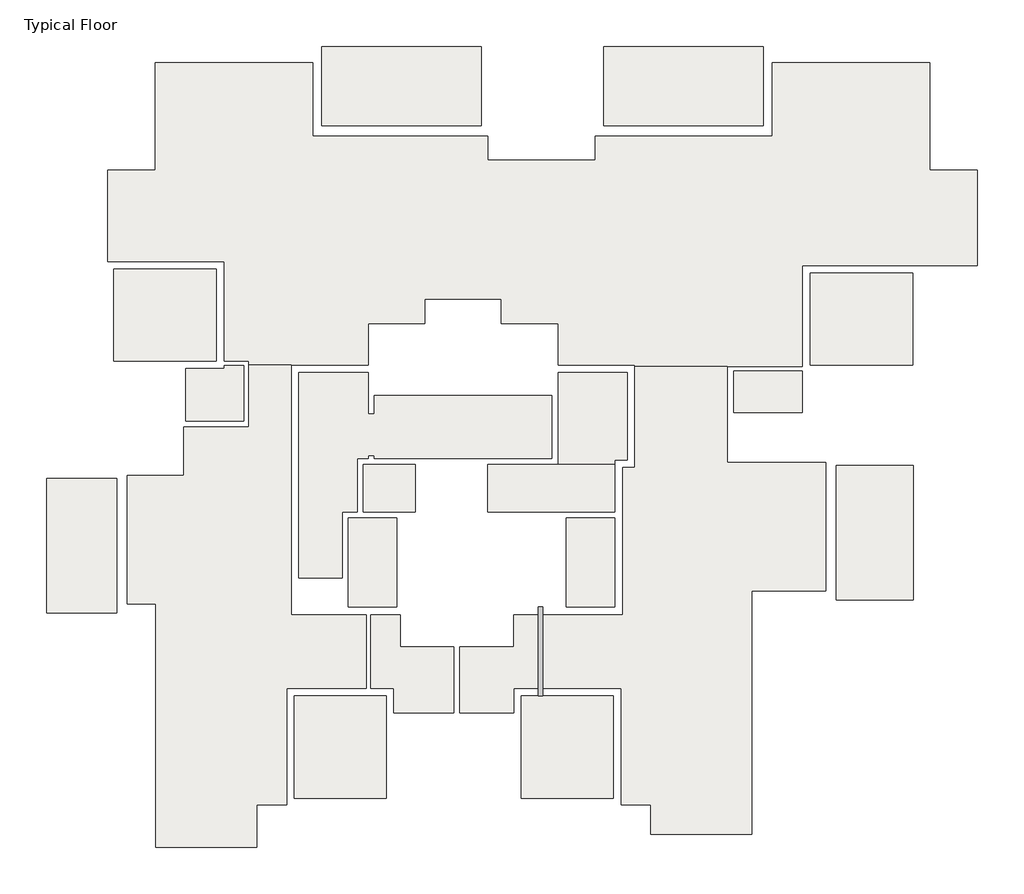
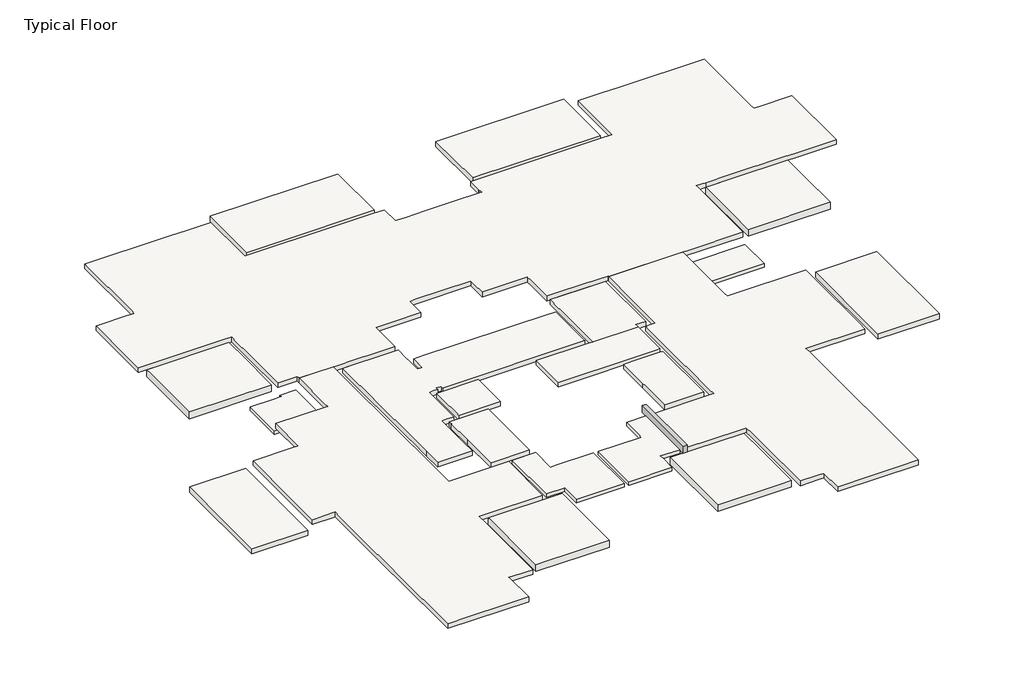
# One storey: 21 slabs, 1 beam.
"""IFC4 building model written with IfcOpenShell, lengths in millimetres."""

from ifc_helpers import new_model, si_unit, frame, origin, place, context, project, spatial, polyline, outline, extrude, faceted_brep, element, save

model = new_model("IFC4")

# Units and contexts
model_context = context("Model", 3, world=origin())
ifc_project = project(units=[si_unit("LENGTHUNIT", "METRE", prefix="MILLI")], contexts=[model_context])

# Site, building, storey
site = spatial("IfcSite", under=ifc_project)
building = spatial("IfcBuilding", under=site)
storey = spatial("IfcBuildingStorey", under=building, Name="Typical Floor", Elevation=3150.0)

# Beam
placement = place(None, origin())
element("IfcBeam", 1, ObjectType="Concrete Rectengular Beam : 15/60", at=placement, inside=storey, context=model_context, shape_type="Brep", body=[
    faceted_brep([(-12635.911942, -10778.5353827, 3450.0), (-12485.911942, -10778.5353827, 3450.0), (-12485.911942, -7874.1201217, 3450.0), (-12635.911942, -7874.1201217, 3450.0), (-12485.911942, -10778.5353827, 3150.0), (-12485.911942, -10528.5353827, 3150.0), (-12485.911942, -10528.5353827, 2950.0), (-12485.911942, -10528.5353827, 2850.0), (-12485.911942, -8124.1201217, 2850.0), (-12485.911942, -8124.1201217, 2950.0), (-12485.911942, -8124.1201217, 3150.0), (-12485.911942, -7874.1201217, 3150.0), (-12635.911942, -10528.5353827, 2850.0), (-12635.911942, -8124.1201217, 2850.0), (-12635.911942, -7874.1201217, 3150.0), (-12635.911942, -8124.1201217, 3150.0), (-12635.911942, -8124.1201217, 3000.0), (-12635.911942, -10528.5353827, 3000.0), (-12635.911942, -10528.5353827, 3150.0), (-12635.911942, -10778.5353827, 3150.0)], [[[0, 1, 2, 3]], [[2, 1, 4, 5, 6, 7, 8, 9, 10, 11]], [[7, 12, 13, 8]], [[0, 3, 14, 15, 16, 13, 12, 17, 18, 19]], [[1, 0, 19, 4]], [[3, 2, 11, 14]], [[5, 18, 17, 12, 7, 6]], [[18, 5, 4, 19]], [[15, 10, 9, 8, 13, 16]], [[10, 15, 14, 11]]]),
])

# Slabs
element("IfcSlab", 2, ObjectType="15", at=placement, inside=storey, context=model_context, shape_type="SweptSolid", body=[
    extrude(outline(polyline([(-3995.4992849, -160.4554551), (-3995.4992849, -1513.3876412), (-6249.3881109, -1513.3876412), (-6249.3881109, -160.4554551), (-3995.4992849, -160.4554551)])), frame((0.0, 0.0, 2550.0), z_axis=(0.0, 0.0, 1.0), x_axis=(1.0, 0.0, 0.0)), (0.0, 0.0, 1.0), 150.0),
])
element("IfcSlab", 3, ObjectType="15", at=placement, inside=storey, context=model_context, shape_type="Brep", body=[
    faceted_brep([(-22902.2127458, -79.7184462, 2550.0), (-22902.2127458, 20.2815538, 2550.0), (-22250.9487358, 20.2815538, 2550.0), (-22250.9487358, -1784.190313, 2550.0), (-24160.0622873, -1784.190313, 2550.0), (-24160.0622873, -79.7184462, 2550.0), (-23152.2127458, -79.7184462, 2550.0), (-22902.2127458, 20.2815538, 2700.0), (-22902.2127458, -79.7184462, 2700.0), (-23152.2127458, -79.7184462, 2700.0), (-24160.0622873, -79.7184462, 2700.0), (-24160.0622873, -1784.190313, 2700.0), (-22250.9487358, -1784.190313, 2700.0), (-22250.9487358, 20.2815538, 2700.0)], [[[0, 1, 2, 3, 4, 5, 6]], [[7, 8, 9, 10, 11, 12, 13]], [[8, 0, 6, 5, 10, 9]], [[1, 0, 8, 7]], [[2, 1, 7, 13]], [[3, 2, 13, 12]], [[4, 3, 12, 11]], [[5, 4, 11, 10]]]),
])
element("IfcSlab", 4, ObjectType="15", at=placement, inside=storey, context=model_context, shape_type="Brep", body=[
    faceted_brep([(-17147.6559701, -8124.1201217, 3000.0), (-17147.6559701, -9176.0843468, 3000.0), (-16947.6559701, -9176.0843468, 3000.0), (-15389.5217009, -9176.0843468, 3000.0), (-15389.5217009, -11338.1261219, 3000.0), (-17348.1541021, -11338.1261219, 3000.0), (-17348.1541021, -10778.5353827, 3000.0), (-17348.1541021, -10528.5353827, 3000.0), (-18103.1541021, -10528.5353827, 3000.0), (-18103.1541021, -8124.1201217, 3000.0), (-17147.6559701, -9176.0843468, 3150.0), (-17147.6559701, -8124.1201217, 3150.0), (-18103.1541021, -8124.1201217, 3150.0), (-18103.1541021, -10528.5353827, 3150.0), (-17348.1541021, -10528.5353827, 3150.0), (-17348.1541021, -10778.5353827, 3150.0), (-17348.1541021, -11338.1261219, 3150.0), (-15389.5217009, -11338.1261219, 3150.0), (-15389.5217009, -9176.0843468, 3150.0), (-16947.6559701, -9176.0843468, 3150.0)], [[[0, 1, 2, 3, 4, 5, 6, 7, 8, 9]], [[10, 11, 12, 13, 14, 15, 16, 17, 18, 19]], [[1, 0, 11, 10]], [[1, 10, 19, 18, 3, 2]], [[4, 3, 18, 17]], [[5, 4, 17, 16]], [[5, 16, 15, 14, 7, 6]], [[8, 7, 14, 13]], [[9, 8, 13, 12]], [[0, 9, 12, 11]]]),
])
element("IfcSlab", 5, ObjectType="15", at=placement, inside=storey, context=model_context, shape_type="Brep", body=[
    faceted_brep([(-12635.911942, -8124.1201217, 3000.0), (-12635.911942, -10528.5353827, 3000.0), (-13430.911942, -10528.5353827, 3000.0), (-13430.911942, -10778.5353827, 3000.0), (-13430.911942, -11338.1261219, 3000.0), (-15189.5217009, -11338.1261219, 3000.0), (-15189.5217009, -9176.0843468, 3000.0), (-13431.410074, -9176.0843468, 3000.0), (-13431.410074, -8976.0843468, 3000.0), (-13431.410074, -8124.1201217, 3000.0), (-12635.911942, -10528.5353827, 3150.0), (-12635.911942, -8124.1201217, 3150.0), (-13431.410074, -8124.1201217, 3150.0), (-13431.410074, -8976.0843468, 3150.0), (-13431.410074, -9176.0843468, 3150.0), (-15189.5217009, -9176.0843468, 3150.0), (-15189.5217009, -11338.1261219, 3150.0), (-13430.911942, -11338.1261219, 3150.0), (-13430.911942, -10778.5353827, 3150.0), (-13430.911942, -10528.5353827, 3150.0)], [[[0, 1, 2, 3, 4, 5, 6, 7, 8, 9]], [[10, 11, 12, 13, 14, 15, 16, 17, 18, 19]], [[1, 0, 11, 10]], [[2, 1, 10, 19]], [[2, 19, 18, 17, 4, 3]], [[5, 4, 17, 16]], [[6, 5, 16, 15]], [[7, 6, 15, 14]], [[7, 14, 13, 12, 9, 8]], [[0, 9, 12, 11]]]),
])
element("IfcSlab", 6, ObjectType="20", at=placement, inside=storey, context=model_context, shape_type="Brep", body=[
    faceted_brep([(-14287.2982207, 7522.5061661, 2950.0), (-14287.2982207, 6745.5504319, 2950.0), (-10767.128403, 6745.5504319, 2950.0), (-10767.128403, 6945.5504319, 2950.0), (-10767.6095532, 6945.5504319, 2950.0), (-10767.6095532, 7522.0250158, 2950.0), (-10278.642045, 7522.0250158, 2950.0), (-7273.2531624, 7522.0250158, 2950.0), (-6464.4905676, 7522.0250158, 2950.0), (-5362.5320031, 7522.0250158, 2950.0), (-4977.1589702, 7522.0250158, 2950.0), (-4977.1589702, 7872.0250158, 2950.0), (-4977.1589702, 9926.4176344, 2950.0), (161.8198592, 9926.4176344, 2950.0), (161.8198592, 6620.0664514, 2950.0), (161.3217272, 6620.0664514, 2950.0), (161.3217272, 6420.0664514, 2950.0), (1724.6637401, 6420.0664514, 2950.0), (1724.6637401, 3294.4013319, 2950.0), (11.338709, 3294.4013319, 2950.0), (-388.661291, 3294.4013319, 2950.0), (-2382.6064399, 3294.4013319, 2950.0), (-2675.3362599, 3294.4013319, 2950.0), (-3574.7135949, 3294.4013319, 2950.0), (-3574.7135949, 3294.8994639, 2950.0), (-3995.4992849, 3294.8994639, 2950.0), (-3995.4992849, 3044.8994639, 2950.0), (-3995.4992849, -10.4554551, 2950.0), (-6449.3881109, -10.4554551, 2950.0), (-9474.5664195, -10.4554551, 2950.0), (-9474.5664195, 39.0464129, 2950.0), (-10476.5363052, 39.0464129, 2950.0), (-11477.9854165, 39.0464129, 2950.0), (-11984.1625168, 39.0464129, 2950.0), (-11984.1625168, 1141.4974488, 2950.0), (-11984.1625168, 1391.4974488, 2950.0), (-13837.0933073, 1391.4974488, 2950.0), (-13837.0933073, 1942.9408995, 2950.0), (-13837.0933073, 2192.9408995, 2950.0), (-16091.0047757, 2192.9408995, 2950.0), (-16341.0047757, 2192.9408995, 2950.0), (-16341.0047757, 1391.4691458, 2950.0), (-17944.4124515, 1391.4691458, 2950.0), (-18194.4124515, 1391.4691458, 2950.0), (-18194.4124515, 39.5388843, 2950.0), (-18915.6849523, 39.5388843, 2950.0), (-19917.1340636, 39.5388843, 2950.0), (-20453.5033605, 39.5388843, 2950.0), (-20703.5033605, 39.5388843, 2950.0), (-22100.9487358, 39.5388843, 2950.0), (-22100.9487358, 170.2815538, 2950.0), (-22902.2127458, 170.2815538, 2950.0), (-22902.2127458, 2208.0433561, 2950.0), (-22902.2127458, 3085.0930561, 2950.0), (-22902.2127458, 3425.0930561, 2950.0), (-23152.2127458, 3425.0930561, 2950.0), (-26709.0507397, 3425.0930561, 2950.0), (-26709.0507397, 6420.0664514, 2950.0), (-26578.3590155, 6420.0664514, 2950.0), (-25426.4061116, 6420.0664514, 2950.0), (-25146.2068588, 6420.0664514, 2950.0), (-25146.2068588, 6620.0664514, 2950.0), (-25146.2068588, 9925.9195024, 2950.0), (-24284.8686951, 9925.9195024, 2950.0), (-22681.9251878, 9925.9195024, 2950.0), (-21629.9609627, 9925.9195024, 2950.0), (-20978.9930017, 9925.9195024, 2950.0), (-20006.7412186, 9925.9195024, 2950.0), (-20006.7412186, 7872.5061661, 2950.0), (-20006.7412186, 7522.5061661, 2950.0), (-19621.8549965, 7522.5061661, 2950.0), (-18519.896432, 7522.5061661, 2950.0), (-17711.1338372, 7522.5061661, 2950.0), (-14706.2657289, 7522.5061661, 2950.0), (-14287.2982207, 6745.5504319, 3150.0), (-14287.2982207, 7522.5061661, 3150.0), (-14706.2657289, 7522.5061661, 3150.0), (-17711.1338372, 7522.5061661, 3150.0), (-18519.896432, 7522.5061661, 3150.0), (-19621.8549965, 7522.5061661, 3150.0), (-20006.7412186, 7522.5061661, 3150.0), (-20006.7412186, 7872.5061661, 3150.0), (-20006.7412186, 9925.9195024, 3150.0), (-20978.9930017, 9925.9195024, 3150.0), (-21629.9609627, 9925.9195024, 3150.0), (-22681.9251878, 9925.9195024, 3150.0), (-24284.8686951, 9925.9195024, 3150.0), (-25146.2068588, 9925.9195024, 3150.0), (-25146.2068588, 6620.0664514, 3150.0), (-25146.2068588, 6420.0664514, 3150.0), (-25426.4061116, 6420.0664514, 3150.0), (-26578.3590155, 6420.0664514, 3150.0), (-26709.0507397, 6420.0664514, 3150.0), (-26709.0507397, 3425.0930561, 3150.0), (-23152.2127458, 3425.0930561, 3150.0), (-22902.2127458, 3425.0930561, 3150.0), (-22902.2127458, 3085.0930561, 3150.0), (-22902.2127458, 2208.0433561, 3150.0), (-22902.2127458, 170.2815538, 3150.0), (-22100.9487358, 170.2815538, 3150.0), (-22100.9487358, 39.5388843, 3150.0), (-20703.5033605, 39.5388843, 3150.0), (-20453.5033605, 39.5388843, 3150.0), (-19917.1340636, 39.5388843, 3150.0), (-18915.6849523, 39.5388843, 3150.0), (-18194.4124515, 39.5388843, 3150.0), (-18194.4124515, 1391.4691458, 3150.0), (-17944.4124515, 1391.4691458, 3150.0), (-16341.0047757, 1391.4691458, 3150.0), (-16341.0047757, 2192.9408995, 3150.0), (-16091.0047757, 2192.9408995, 3150.0), (-13837.0933073, 2192.9408995, 3150.0), (-13837.0933073, 1942.9408995, 3150.0), (-13837.0933073, 1391.4974488, 3150.0), (-11984.1625168, 1391.4974488, 3150.0), (-11984.1625168, 1141.4974488, 3150.0), (-11984.1625168, 39.0464129, 3150.0), (-11477.9854165, 39.0464129, 3150.0), (-10476.5363052, 39.0464129, 3150.0), (-9474.5664195, 39.0464129, 3150.0), (-9474.5664195, -10.4554551, 3150.0), (-6449.3881109, -10.4554551, 3150.0), (-6249.3881109, -10.4554551, 3150.0), (-3995.4992849, -10.4554551, 3150.0), (-3995.4992849, 3044.8994639, 3150.0), (-3995.4992849, 3294.8994639, 3150.0), (-3574.7135949, 3294.8994639, 3150.0), (-3574.7135949, 3294.4013319, 3150.0), (-2675.3362599, 3294.4013319, 3150.0), (-388.661291, 3294.4013319, 3150.0), (11.338709, 3294.4013319, 3150.0), (1724.6637401, 3294.4013319, 3150.0), (1724.6637401, 6420.0664514, 3150.0), (1593.9720159, 6420.0664514, 3150.0), (442.019112, 6420.0664514, 3150.0), (161.3217272, 6420.0664514, 3150.0), (161.3217272, 6620.0664514, 3150.0), (161.8198592, 6620.0664514, 3150.0), (161.8198592, 9926.4176344, 3150.0), (-700.0390789, 9926.4176344, 3150.0), (-2302.4618118, 9926.4176344, 3150.0), (-3354.4260369, 9926.4176344, 3150.0), (-4005.3939979, 9926.4176344, 3150.0), (-4977.1589702, 9926.4176344, 3150.0), (-4977.1589702, 7872.0250158, 3150.0), (-4977.1589702, 7522.0250158, 3150.0), (-5362.5320031, 7522.0250158, 3150.0), (-6464.4905676, 7522.0250158, 3150.0), (-7273.2531624, 7522.0250158, 3150.0), (-10278.642045, 7522.0250158, 3150.0), (-10767.6095532, 7522.0250158, 3150.0), (-10767.6095532, 6945.5504319, 3150.0), (-10767.128403, 6945.5504319, 3150.0), (-10767.128403, 6745.5504319, 3150.0), (-11941.4746047, 6745.5504319, 3150.0), (-13043.4331692, 6745.5504319, 3150.0), (-13867.2982207, 6745.5504319, 3150.0), (-3574.7135949, 3294.4013319, 3100.0)], [[[0, 1, 2, 3, 4, 5, 6, 7, 8, 9, 10, 11, 12, 13, 14, 15, 16, 17, 18, 19, 20, 21, 22, 23, 24, 25, 26, 27, 28, 29, 30, 31, 32, 33, 34, 35, 36, 37, 38, 39, 40, 41, 42, 43, 44, 45, 46, 47, 48, 49, 50, 51, 52, 53, 54, 55, 56, 57, 58, 59, 60, 61, 62, 63, 64, 65, 66, 67, 68, 69, 70, 71, 72, 73]], [[74, 75, 76, 77, 78, 79, 80, 81, 82, 83, 84, 85, 86, 87, 88, 89, 90, 91, 92, 93, 94, 95, 96, 97, 98, 99, 100, 101, 102, 103, 104, 105, 106, 107, 108, 109, 110, 111, 112, 113, 114, 115, 116, 117, 118, 119, 120, 121, 122, 123, 124, 125, 126, 127, 128, 129, 130, 131, 132, 133, 134, 135, 136, 137, 138, 139, 140, 141, 142, 143, 144, 145, 146, 147, 148, 149, 150, 151, 152, 153, 154, 155, 156]], [[89, 60, 59, 58, 57, 92, 91, 90]], [[60, 89, 88, 87, 62, 61]], [[62, 87, 86, 85, 84, 83, 82, 67, 66, 65, 64, 63]], [[67, 82, 81, 80, 69, 68]], [[69, 80, 79, 78, 77, 76, 75, 0, 73, 72, 71, 70]], [[1, 0, 75, 74]], [[1, 74, 156, 155, 154, 153, 2]], [[150, 5, 4, 151]], [[6, 5, 150, 149]], [[6, 149, 148, 147, 146, 145, 10, 9, 8, 7]], [[10, 145, 144, 143, 12, 11]], [[13, 12, 143, 142, 141, 140, 139, 138]], [[13, 138, 137, 14]], [[132, 17, 16, 135, 134, 133]], [[18, 17, 132, 131]], [[18, 131, 130, 129, 128, 127, 157, 23, 22, 21, 20, 19]], [[123, 27, 26, 25, 125, 124]], [[28, 27, 123, 122, 121]], [[29, 28, 121, 120]], [[30, 29, 120, 119]], [[30, 119, 118, 117, 116, 33, 32, 31]], [[33, 116, 115, 114, 35, 34]], [[36, 35, 114, 113]], [[36, 113, 112, 111, 38, 37]], [[38, 111, 110, 109, 40, 39]], [[41, 40, 109, 108]], [[41, 108, 107, 106, 43, 42]], [[44, 43, 106, 105]], [[44, 105, 104, 103, 102, 101, 48, 47, 46, 45]], [[49, 48, 101, 100]], [[50, 49, 100, 99]], [[51, 50, 99, 98]], [[51, 98, 97, 96, 95, 54, 53, 52]], [[54, 95, 94, 93, 56, 55]], [[57, 56, 93, 92]], [[24, 126, 125, 25]], [[126, 24, 23, 157, 127]], [[3, 152, 151, 4]], [[2, 153, 152, 3]], [[136, 15, 14, 137]], [[135, 16, 15, 136]]]),
])
element("IfcSlab", 7, ObjectType="20", at=placement, inside=storey, context=model_context, shape_type="Brep", body=[
    faceted_brep([(-3237.9389996, -3145.5397979, 2950.0), (-3237.9389996, -7343.0129016, 2950.0), (-5648.4371316, -7343.0129016, 2950.0), (-5648.4371316, -7643.0129016, 2950.0), (-5648.4371316, -8389.7150498, 2950.0), (-5648.4371316, -9591.6622931, 2950.0), (-5648.4371316, -11149.2984303, 2950.0), (-5648.4371316, -11806.6175745, 2950.0), (-5648.4371316, -15307.4032645, 2950.0), (-8953.7920507, -15307.4032645, 2950.0), (-8953.7920507, -14334.8752446, 2950.0), (-9153.7920507, -14334.8752446, 2950.0), (-9925.0588909, -14334.8752446, 2950.0), (-9925.0588909, -11794.8752446, 2950.0), (-9925.0588909, -10898.8059589, 2950.0), (-9925.0588909, -10528.5353827, 2950.0), (-10175.0588909, -10528.5353827, 2950.0), (-12485.911942, -10528.5353827, 2950.0), (-12485.911942, -8124.1201217, 2950.0), (-9876.055155, -8124.1201217, 2950.0), (-9876.055155, -7874.1201217, 2950.0), (-9876.055155, -4468.2840524, 2950.0), (-9876.055155, -3466.3141668, 2950.0), (-9876.055155, -3316.3311485, 2950.0), (-9724.5664195, -3316.3311485, 2950.0), (-9474.5664195, -3316.3311485, 2950.0), (-9474.5664195, -210.9535871, 2950.0), (-9474.5664195, -10.4554551, 2950.0), (-6449.3881109, -10.4554551, 2950.0), (-6449.3881109, -1513.3876412, 2950.0), (-6449.3881109, -1713.3876412, 2950.0), (-6449.3881109, -2845.5511191, 2950.0), (-6449.3881109, -3145.5397979, 2950.0), (-6249.3881109, -3145.5397979, 2950.0), (-3237.9389996, -7343.0129016, 3150.0), (-3237.9389996, -6903.0129016, 3150.0), (-3237.9389996, -3892.3076005, 3150.0), (-3237.9389996, -3145.5397979, 3150.0), (-6249.3881109, -3145.5397979, 3150.0), (-6449.3881109, -3145.5397979, 3150.0), (-6449.3881109, -2845.5511191, 3150.0), (-6449.3881109, -1713.3876412, 3150.0), (-6449.3881109, -1513.3876412, 3150.0), (-6449.3881109, -10.4554551, 3150.0), (-9474.5664195, -10.4554551, 3150.0), (-9474.5664195, -210.9535871, 3150.0), (-9474.5664195, -3316.3311485, 3150.0), (-9724.5664195, -3316.3311485, 3150.0), (-9876.055155, -3316.3311485, 3150.0), (-9876.055155, -3466.3141668, 3150.0), (-9876.055155, -4468.2840524, 3150.0), (-9876.055155, -7874.1201217, 3150.0), (-9876.055155, -8124.1201217, 3150.0), (-12485.911942, -8124.1201217, 3150.0), (-12485.911942, -10528.5353827, 3150.0), (-10175.0588909, -10528.5353827, 3150.0), (-9925.0588909, -10528.5353827, 3150.0), (-9925.0588909, -10898.8059589, 3150.0), (-9925.0588909, -11794.8752446, 3150.0), (-9925.0588909, -14334.8752446, 3150.0), (-9153.7920507, -14334.8752446, 3150.0), (-8953.7920507, -14334.8752446, 3150.0), (-8953.7920507, -15307.4032645, 3150.0), (-8093.7920507, -15307.4032645, 3150.0), (-6499.9032247, -15307.4032645, 3150.0), (-5648.4371316, -15307.4032645, 3150.0), (-5648.4371316, -11806.6175745, 3150.0), (-5648.4371316, -11149.2984303, 3150.0), (-5648.4371316, -9591.6622931, 3150.0), (-5648.4371316, -8389.7150498, 3150.0), (-5648.4371316, -7643.0129016, 3150.0), (-5648.4371316, -7343.0129016, 3150.0)], [[[0, 1, 2, 3, 4, 5, 6, 7, 8, 9, 10, 11, 12, 13, 14, 15, 16, 17, 18, 19, 20, 21, 22, 23, 24, 25, 26, 27, 28, 29, 30, 31, 32, 33]], [[34, 35, 36, 37, 38, 39, 40, 41, 42, 43, 44, 45, 46, 47, 48, 49, 50, 51, 52, 53, 54, 55, 56, 57, 58, 59, 60, 61, 62, 63, 64, 65, 66, 67, 68, 69, 70, 71]], [[39, 32, 31, 30, 29, 28, 43, 42, 41, 40]], [[32, 39, 38, 37, 0, 33]], [[1, 0, 37, 36, 35, 34]], [[2, 1, 34, 71]], [[2, 71, 70, 69, 68, 67, 66, 65, 8, 7, 6, 5, 4, 3]], [[9, 8, 65, 64, 63, 62]], [[10, 9, 62, 61]], [[10, 61, 60, 59, 12, 11]], [[12, 59, 58, 57, 56, 15, 14, 13]], [[15, 56, 55, 54, 17, 16]], [[18, 17, 54, 53]], [[19, 18, 53, 52]], [[19, 52, 51, 50, 49, 48, 23, 22, 21, 20]], [[23, 48, 47, 46, 25, 24]], [[25, 46, 45, 44, 27, 26]], [[28, 27, 44, 43]]]),
])
element("IfcSlab", 8, ObjectType="20", at=placement, inside=storey, context=model_context, shape_type="Brep", body=[
    faceted_brep([(-18253.1541021, -8124.1201217, 2950.0), (-18253.1541021, -10528.5353827, 2950.0), (-20604.0071531, -10528.5353827, 2950.0), (-20854.0071531, -10528.5353827, 2950.0), (-20854.0071531, -10898.8059589, 2950.0), (-20854.0071531, -11794.8752446, 2950.0), (-20854.0071531, -14334.8752446, 2950.0), (-21625.2739934, -14334.8752446, 2950.0), (-21825.2739934, -14334.8752446, 2950.0), (-21825.2739934, -15727.4032645, 2950.0), (-25131.1270445, -15727.4032645, 2950.0), (-25131.1270445, -12221.0520814, 2950.0), (-25131.1270445, -11570.0841204, 2950.0), (-25131.1270445, -10012.4479831, 2950.0), (-25131.1270445, -8810.5007399, 2950.0), (-25131.1270445, -8064.2310693, 2950.0), (-25131.1270445, -7764.2310693, 2950.0), (-26062.7923903, -7764.2310693, 2950.0), (-26062.7923903, -3566.82362, 2950.0), (-24415.0622873, -3566.82362, 2950.0), (-24215.0622873, -3566.82362, 2950.0), (-24215.0622873, -1984.190313, 2950.0), (-22100.9487358, -1984.190313, 2950.0), (-22100.9487358, -1784.190313, 2950.0), (-22100.9487358, 39.5388843, 2950.0), (-20703.5033605, 39.5388843, 2950.0), (-20703.5033605, -5109.3573005, 2950.0), (-20703.0108891, -5109.3573005, 2950.0), (-20703.0108891, -6110.8064118, 2950.0), (-20703.0108891, -7874.1201217, 2950.0), (-20703.5033605, -7874.1201217, 2950.0), (-20703.5033605, -8124.1201217, 2950.0), (-18253.1541021, -10528.5353827, 3150.0), (-18253.1541021, -8124.1201217, 3150.0), (-20703.5033605, -8124.1201217, 3150.0), (-20703.5033605, -7874.1201217, 3150.0), (-20703.0108891, -7874.1201217, 3150.0), (-20703.0108891, -6110.8064118, 3150.0), (-20703.0108891, -5109.3573005, 3150.0), (-20703.5033605, -5109.3573005, 3150.0), (-20703.5033605, 39.5388843, 3150.0), (-22100.9487358, 39.5388843, 3150.0), (-22100.9487358, -1784.190313, 3150.0), (-22100.9487358, -1984.190313, 3150.0), (-24215.0622873, -1984.190313, 3150.0), (-24215.0622873, -3566.82362, 3150.0), (-24415.0622873, -3566.82362, 3150.0), (-26062.7923903, -3566.82362, 3150.0), (-26062.7923903, -4267.7859204, 3150.0), (-26062.7923903, -7272.6540287, 3150.0), (-26062.7923903, -7764.2310693, 3150.0), (-25131.1270445, -7764.2310693, 3150.0), (-25131.1270445, -8064.2310693, 3150.0), (-25131.1270445, -8810.5007399, 3150.0), (-25131.1270445, -10012.4479831, 3150.0), (-25131.1270445, -11570.0841204, 3150.0), (-25131.1270445, -12221.0520814, 3150.0), (-25131.1270445, -15727.4032645, 3150.0), (-24279.6609514, -15727.4032645, 3150.0), (-22676.7174441, -15727.4032645, 3150.0), (-21825.2739934, -15727.4032645, 3150.0), (-21825.2739934, -14334.8752446, 3150.0), (-21625.2739934, -14334.8752446, 3150.0), (-20854.0071531, -14334.8752446, 3150.0), (-20854.0071531, -11794.8752446, 3150.0), (-20854.0071531, -10898.8059589, 3150.0), (-20854.0071531, -10528.5353827, 3150.0), (-20604.0071531, -10528.5353827, 3150.0), (-20703.0108891, -5109.3573005, 3050.0)], [[[0, 1, 2, 3, 4, 5, 6, 7, 8, 9, 10, 11, 12, 13, 14, 15, 16, 17, 18, 19, 20, 21, 22, 23, 24, 25, 26, 27, 28, 29, 30, 31]], [[32, 33, 34, 35, 36, 37, 38, 39, 40, 41, 42, 43, 44, 45, 46, 47, 48, 49, 50, 51, 52, 53, 54, 55, 56, 57, 58, 59, 60, 61, 62, 63, 64, 65, 66, 67]], [[24, 41, 40, 25]], [[36, 29, 28, 27, 68, 38, 37]], [[33, 0, 31, 34]], [[1, 0, 33, 32]], [[1, 32, 67, 66, 3, 2]], [[3, 66, 65, 64, 63, 6, 5, 4]], [[6, 63, 62, 61, 8, 7]], [[9, 8, 61, 60]], [[10, 9, 60, 59, 58, 57]], [[10, 57, 56, 55, 54, 53, 52, 51, 16, 15, 14, 13, 12, 11]], [[17, 16, 51, 50]], [[18, 17, 50, 49, 48, 47]], [[18, 47, 46, 45, 20, 19]], [[21, 20, 45, 44]], [[22, 21, 44, 43]], [[22, 43, 42, 41, 24, 23]], [[35, 30, 29, 36]], [[34, 31, 30, 35]], [[39, 26, 25, 40]], [[26, 39, 38, 68, 27]]]),
])
element("IfcSlab", 9, ObjectType="20", at=placement, inside=storey, context=model_context, shape_type="Brep", body=[
    faceted_brep([(-20453.5033605, -210.4611157, 2950.0), (-18194.4124515, -210.4611157, 2950.0), (-18194.4124515, -762.4310014, 2950.0), (-18194.4124515, -962.4310014, 2950.0), (-18194.4124515, -1563.404623, 2950.0), (-17994.4124515, -1563.404623, 2950.0), (-17994.4124515, -962.4325886, 2950.0), (-17984.178103, -962.4325886, 2950.0), (-17593.4388298, -962.4325886, 2950.0), (-16290.9821333, -962.4325886, 2950.0), (-15740.0028511, -962.4325886, 2950.0), (-14438.066929, -962.4325886, 2950.0), (-13887.0876467, -962.4325886, 2950.0), (-12584.1498, -962.4325886, 2950.0), (-12184.178103, -962.4325886, 2950.0), (-12184.178103, -3015.8216954, 2950.0), (-17993.9143195, -3015.8216954, 2950.0), (-17993.9143195, -2915.3348845, 2950.0), (-18193.9143195, -2915.3348845, 2950.0), (-18193.9143195, -3015.8216954, 2950.0), (-18350.1013454, -3015.8216954, 2950.0), (-18550.1013454, -3015.8216954, 2950.0), (-18550.1013454, -3666.8122988, 2950.0), (-18550.1013454, -4618.2670707, 2950.0), (-18550.1013454, -4768.7708633, 2950.0), (-18843.2746727, -4768.7708633, 2950.0), (-19043.2746727, -4768.7708633, 2950.0), (-19043.2746727, -5119.2520135, 2950.0), (-19043.2746727, -6221.210578, 2950.0), (-19043.2746727, -6922.1728784, 2950.0), (-20453.0108891, -6922.1728784, 2950.0), (-20453.0108891, -6110.8064118, 2950.0), (-20453.5033605, -6110.8064118, 2950.0), (-20453.5033605, -5109.3573005, 2950.0), (-20453.5033605, -4948.7708633, 2950.0), (-18194.4124515, -210.4611157, 3150.0), (-18915.6849523, -210.4611157, 3150.0), (-19917.1340636, -210.4611157, 3150.0), (-20453.5033605, -210.4611157, 3150.0), (-20453.5033605, -5109.3573005, 3150.0), (-20453.5033605, -6110.8064118, 3150.0), (-20453.0108891, -6110.8064118, 3150.0), (-20453.0108891, -6922.1728784, 3150.0), (-19043.2746727, -6922.1728784, 3150.0), (-19043.2746727, -6221.210578, 3150.0), (-19043.2746727, -5119.2520135, 3150.0), (-19043.2746727, -4768.7708633, 3150.0), (-18843.2746727, -4768.7708633, 3150.0), (-18550.1013454, -4768.7708633, 3150.0), (-18550.1013454, -4618.2670707, 3150.0), (-18550.1013454, -3666.8122988, 3150.0), (-18550.1013454, -3015.8216954, 3150.0), (-18350.1013454, -3015.8216954, 3150.0), (-18193.9143195, -3015.8216954, 3150.0), (-18193.9143195, -2915.3348845, 3150.0), (-17993.9143195, -2915.3348845, 3150.0), (-17993.9143195, -3015.8216954, 3150.0), (-12184.178103, -3015.8216954, 3150.0), (-12184.178103, -2915.3348845, 3150.0), (-12184.178103, -1563.404623, 3150.0), (-12184.178103, -962.4325886, 3150.0), (-12584.1498, -962.4325886, 3150.0), (-13887.0876467, -962.4325886, 3150.0), (-14438.066929, -962.4325886, 3150.0), (-15740.0028511, -962.4325886, 3150.0), (-16290.9821333, -962.4325886, 3150.0), (-17593.4388298, -962.4325886, 3150.0), (-17984.178103, -962.4325886, 3150.0), (-17994.4124515, -962.4325886, 3150.0), (-17994.4124515, -1563.404623, 3150.0), (-18194.4124515, -1563.404623, 3150.0), (-18194.4124515, -962.4310014, 3150.0), (-18194.4124515, -762.4310014, 3150.0), (-20453.5033605, -6110.8064118, 3050.0)], [[[0, 1, 2, 3, 4, 5, 6, 7, 8, 9, 10, 11, 12, 13, 14, 15, 16, 17, 18, 19, 20, 21, 22, 23, 24, 25, 26, 27, 28, 29, 30, 31, 32, 33, 34]], [[35, 36, 37, 38, 39, 40, 41, 42, 43, 44, 45, 46, 47, 48, 49, 50, 51, 52, 53, 54, 55, 56, 57, 58, 59, 60, 61, 62, 63, 64, 65, 66, 67, 68, 69, 70, 71, 72]], [[29, 43, 42, 30]], [[38, 0, 34, 33, 32, 73, 40, 39]], [[1, 0, 38, 37, 36, 35]], [[1, 35, 72, 71, 70, 4, 3, 2]], [[5, 4, 70, 69]], [[6, 5, 69, 68]], [[7, 6, 68, 67]], [[7, 67, 66, 65, 64, 63, 62, 61, 60, 14, 13, 12, 11, 10, 9, 8]], [[15, 14, 60, 59, 58, 57]], [[16, 15, 57, 56]], [[17, 16, 56, 55]], [[18, 17, 55, 54]], [[19, 18, 54, 53]], [[19, 53, 52, 51, 21, 20]], [[21, 51, 50, 49, 48, 24, 23, 22]], [[24, 48, 47, 46, 26, 25]], [[26, 46, 45, 44, 43, 29, 28, 27]], [[41, 31, 30, 42]], [[31, 41, 40, 73, 32]]]),
])
element("IfcSlab", 10, ObjectType="20", at=placement, inside=storey, context=model_context, shape_type="Brep", body=[
    faceted_brep([(-16646.6710273, -3215.8216954, 2950.0), (-16646.6710273, -4768.7708633, 2950.0), (-18350.1013454, -4768.7708633, 2950.0), (-18350.1013454, -3215.8216954, 2950.0), (-16646.6710273, -4768.7708633, 3150.0), (-16646.6710273, -3215.8216954, 3150.0), (-18350.1013454, -3215.8216954, 3150.0), (-18350.1013454, -3666.8122988, 3150.0), (-18350.1013454, -4618.2670707, 3150.0), (-18350.1013454, -4768.7708633, 3150.0)], [[[0, 1, 2, 3]], [[4, 5, 6, 7, 8, 9]], [[1, 0, 5, 4]], [[2, 1, 4, 9]], [[3, 2, 9, 8, 7, 6]], [[0, 3, 6, 5]]]),
])
element("IfcSlab", 11, ObjectType="20", at=placement, inside=storey, context=model_context, shape_type="Brep", body=[
    faceted_brep([(-11723.2701442, -4968.7708633, 2950.0), (-10126.055155, -4968.7708633, 2950.0), (-10126.055155, -7874.1201217, 2950.0), (-11723.2701442, -7874.1201217, 2950.0), (-11723.2701442, -6321.6973888, 2950.0), (-10126.055155, -4968.7708633, 3150.0), (-10226.0438338, -4968.7708633, 3150.0), (-11328.0023982, -4968.7708633, 3150.0), (-11723.2701442, -4968.7708633, 3150.0), (-11723.2701442, -6321.6973888, 3150.0), (-11723.2701442, -6521.6973888, 3150.0), (-11723.2701442, -7874.1201217, 3150.0), (-10126.055155, -7874.1201217, 3150.0)], [[[0, 1, 2, 3, 4]], [[5, 6, 7, 8, 9, 10, 11, 12]], [[1, 0, 8, 7, 6, 5]], [[2, 1, 5, 12]], [[3, 2, 12, 11]], [[4, 3, 11, 10, 9]], [[0, 4, 9, 8]]]),
])
element("IfcSlab", 12, ObjectType="20", at=placement, inside=storey, context=model_context, shape_type="Brep", body=[
    faceted_brep([(-17252.8523926, -4968.7708633, 2950.0), (-17252.8523926, -7874.1201217, 2950.0), (-18843.2746727, -7874.1201217, 2950.0), (-18843.2746727, -6221.210578, 2950.0), (-18848.2746727, -6221.210578, 2950.0), (-18848.2746727, -5119.2520135, 2950.0), (-18843.2746727, -5119.2520135, 2950.0), (-18843.2746727, -4968.7708633, 2950.0), (-17252.8523926, -7874.1201217, 3150.0), (-17252.8523926, -4968.7708633, 3150.0), (-18843.2746727, -4968.7708633, 3150.0), (-18843.2746727, -5119.2520135, 3150.0), (-18848.2746727, -5119.2520135, 3150.0), (-18848.2746727, -6221.210578, 3150.0), (-18843.2746727, -6221.210578, 3150.0), (-18843.2746727, -7874.1201217, 3150.0), (-18848.2746727, -5119.2520135, 3050.0), (-18848.2746727, -6221.210578, 3050.0)], [[[0, 1, 2, 3, 4, 5, 6, 7]], [[8, 9, 10, 11, 12, 13, 14, 15]], [[1, 0, 9, 8]], [[1, 8, 15, 2]], [[12, 16, 5, 4, 17, 13]], [[9, 0, 7, 10]], [[6, 11, 10, 7]], [[11, 6, 5, 16, 12]], [[14, 3, 2, 15]], [[3, 14, 13, 17, 4]]]),
])
element("IfcSlab", 13, ObjectType="20", at=placement, inside=storey, context=model_context, shape_type="Brep", body=[
    faceted_brep([(-14282.8761671, -3215.8216954, 2950.0), (-11984.178103, -3215.8216954, 2950.0), (-10126.055155, -3215.8216954, 2950.0), (-10126.055155, -4768.7708633, 2950.0), (-14282.8761671, -4768.7708633, 2950.0), (-10126.055155, -3215.8216954, 3150.0), (-11984.178103, -3215.8216954, 3150.0), (-12184.178103, -3215.8216954, 3150.0), (-14282.8761671, -3215.8216954, 3150.0), (-14282.8761671, -4768.7708633, 3150.0), (-11328.0023982, -4768.7708633, 3150.0), (-10226.0438338, -4768.7708633, 3150.0), (-10126.055155, -4768.7708633, 3150.0), (-10126.055155, -4468.2840524, 3150.0), (-10126.055155, -3466.3141668, 3150.0), (-10126.055155, -3316.3311485, 3150.0)], [[[0, 1, 2, 3, 4]], [[5, 6, 7, 8, 9, 10, 11, 12, 13, 14, 15]], [[2, 1, 0, 8, 7, 6, 5]], [[3, 2, 5, 15, 14, 13, 12]], [[4, 3, 12, 11, 10, 9]], [[0, 4, 9, 8]]]),
])
element("IfcSlab", 14, ObjectType="20", at=placement, inside=storey, context=model_context, shape_type="Brep", body=[
    faceted_brep([(-11984.178103, -210.9535871, 2950.0), (-9724.5664195, -210.9535871, 2950.0), (-9724.5664195, -3066.3311485, 2950.0), (-10126.055155, -3066.3311485, 2950.0), (-10126.055155, -3215.8216954, 2950.0), (-11984.178103, -3215.8216954, 2950.0), (-9724.5664195, -210.9535871, 3150.0), (-10476.5363052, -210.9535871, 3150.0), (-11477.9854165, -210.9535871, 3150.0), (-11984.178103, -210.9535871, 3150.0), (-11984.178103, -762.4325886, 3150.0), (-11984.178103, -962.4325886, 3150.0), (-11984.178103, -1563.404623, 3150.0), (-11984.178103, -2915.3348845, 3150.0), (-11984.178103, -3215.8216954, 3150.0), (-10126.055155, -3215.8216954, 3150.0), (-10126.055155, -3066.3311485, 3150.0), (-9724.5664195, -3066.3311485, 3150.0)], [[[0, 1, 2, 3, 4, 5]], [[6, 7, 8, 9, 10, 11, 12, 13, 14, 15, 16, 17]], [[1, 0, 9, 8, 7, 6]], [[2, 1, 6, 17]], [[3, 2, 17, 16]], [[4, 3, 16, 15]], [[5, 4, 15, 14]], [[0, 5, 14, 13, 12, 11, 10, 9]]]),
])
element("IfcSlab", 15, ObjectType="23", at=placement, inside=storey, context=model_context, shape_type="SweptSolid", body=[
    extrude(outline(polyline([(-14495.8728839, 10453.9847124), (-14495.8728839, 7872.5061661), (-19706.7412186, 7872.5061661), (-19706.7412186, 10453.9847124), (-14495.8728839, 10453.9847124)])), frame((0.0, 0.0, 2770.0), z_axis=(0.0, 0.0, 1.0), x_axis=(1.0, 0.0, 0.0)), (0.0, 0.0, 1.0), 230.0),
])
element("IfcSlab", 16, ObjectType="23", at=placement, inside=storey, context=model_context, shape_type="SweptSolid", body=[
    extrude(outline(polyline([(-5277.645781, 7872.5061661), (-10489.03489, 7872.5061661), (-10489.03489, 10457.630133), (-5277.645781, 10457.630133), (-5277.645781, 7872.5061661)])), frame((0.0, 0.0, 2770.0), z_axis=(0.0, 0.0, 1.0), x_axis=(1.0, 0.0, 0.0)), (0.0, 0.0, 1.0), 230.0),
])
element("IfcSlab", 17, ObjectType="23", at=placement, inside=storey, context=model_context, shape_type="SweptSolid", body=[
    extrude(outline(polyline([(-28703.6934128, -8064.2310693), (-28703.6934128, -3666.82362), (-26412.7923903, -3666.82362), (-26412.7923903, -8064.2310693), (-28703.6934128, -8064.2310693)])), frame((0.0, 0.0, 2770.0), z_axis=(0.0, 0.0, 1.0), x_axis=(1.0, 0.0, 0.0)), (0.0, 0.0, 1.0), 230.0),
])
element("IfcSlab", 18, ObjectType="23", at=placement, inside=storey, context=model_context, shape_type="SweptSolid", body=[
    extrude(outline(polyline([(-380.3567978, -3245.5397979), (-380.3567978, -7643.0129016), (-2887.9389996, -7643.0129016), (-2887.9389996, -3245.5397979), (-380.3567978, -3245.5397979)])), frame((0.0, 0.0, 2770.0), z_axis=(0.0, 0.0, 1.0), x_axis=(1.0, 0.0, 0.0)), (0.0, 0.0, 1.0), 230.0),
])
element("IfcSlab", 19, ObjectType="29", at=placement, inside=storey, context=model_context, shape_type="Brep", body=[
    faceted_brep([(-23152.2127458, 3175.0930561, 2860.0), (-23152.2127458, 170.2815538, 2860.0), (-26509.0507397, 170.2815538, 2860.0), (-26509.0507397, 3175.0930561, 2860.0), (-23152.2127458, 170.2815538, 3150.0), (-23152.2127458, 2208.0433561, 3150.0), (-23152.2127458, 3085.0930561, 3150.0), (-23152.2127458, 3175.0930561, 3150.0), (-26509.0507397, 3175.0930561, 3150.0), (-26509.0507397, 2974.1024527, 3150.0), (-26509.0507397, 1972.6533414, 3150.0), (-26509.0507397, 170.2815538, 3150.0)], [[[0, 1, 2, 3]], [[4, 5, 6, 7, 8, 9, 10, 11]], [[1, 0, 7, 6, 5, 4]], [[2, 1, 4, 11]], [[3, 2, 11, 10, 9, 8]], [[0, 3, 8, 7]]]),
])
element("IfcSlab", 20, ObjectType="29", at=placement, inside=storey, context=model_context, shape_type="Brep", body=[
    faceted_brep([(-388.661291, 39.0464129, 2860.0), (-3745.4992849, 39.0464129, 2860.0), (-3745.4992849, 3044.8994639, 2860.0), (-2675.3362599, 3044.8994639, 2860.0), (-2675.3362599, 3044.4013319, 2860.0), (-388.661291, 3044.4013319, 2860.0), (-3745.4992849, 39.0464129, 3150.0), (-388.661291, 39.0464129, 3150.0), (-388.661291, 1842.4597492, 3150.0), (-388.661291, 3044.4013319, 3150.0), (-2675.3362599, 3044.4013319, 3150.0), (-2675.3362599, 3044.8994639, 3150.0), (-3574.7135949, 3044.8994639, 3150.0), (-3745.4992849, 3044.8994639, 3150.0), (-2675.3362599, 3044.8994639, 3100.0)], [[[0, 1, 2, 3, 4, 5]], [[6, 7, 8, 9, 10, 11, 12, 13]], [[7, 0, 5, 9, 8]], [[1, 0, 7, 6]], [[2, 1, 6, 13]], [[2, 13, 12, 11, 14, 3]], [[4, 10, 9, 5]], [[10, 4, 3, 14, 11]]]),
])
element("IfcSlab", 21, ObjectType="29", at=placement, inside=storey, context=model_context, shape_type="Brep", body=[
    faceted_brep([(-17598.1541021, -10778.5353827, 2860.0), (-17598.1541021, -14134.8752446, 2860.0), (-20604.0071531, -14134.8752446, 2860.0), (-20604.0071531, -10778.5353827, 2860.0), (-17598.1541021, -14134.8752446, 3150.0), (-17598.1541021, -10778.5353827, 3150.0), (-20604.0071531, -10778.5353827, 3150.0), (-20604.0071531, -10898.8059589, 3150.0), (-20604.0071531, -11794.8752446, 3150.0), (-20604.0071531, -14134.8752446, 3150.0), (-20132.7346523, -14134.8752446, 3150.0), (-19133.1541021, -14134.8752446, 3150.0)], [[[0, 1, 2, 3]], [[4, 5, 6, 7, 8, 9, 10, 11]], [[1, 0, 5, 4]], [[2, 1, 4, 11, 10, 9]], [[3, 2, 9, 8, 7, 6]], [[0, 3, 6, 5]]]),
])
element("IfcSlab", 22, ObjectType="29", at=placement, inside=storey, context=model_context, shape_type="Brep", body=[
    faceted_brep([(-10175.0588909, -10778.5353827, 2860.0), (-10175.0588909, -14134.8526022, 2860.0), (-13180.911942, -14134.8526022, 2860.0), (-13180.911942, -10778.5353827, 2860.0), (-10175.0588909, -14134.8526022, 3150.0), (-10175.0588909, -11794.8752446, 3150.0), (-10175.0588909, -10898.8059589, 3150.0), (-10175.0588909, -10778.5353827, 3150.0), (-13180.911942, -10778.5353827, 3150.0), (-13180.911942, -14134.8526022, 3150.0), (-10646.8295238, -14134.8526022, 3150.0)], [[[0, 1, 2, 3]], [[4, 5, 6, 7, 8, 9, 10]], [[1, 0, 7, 6, 5, 4]], [[2, 1, 4, 10, 9]], [[3, 2, 9, 8]], [[0, 3, 8, 7]]]),
])

save(model, "model.ifc")

# Revit data of these elements
# Type "Concrete Rectengular Beam : 15/60"
#   Length [instance default] = 152.4 cm
#   b = 15 cm
#   h = 60 cm
#   Structural Material [instance default] = Concrete
#   Assembly Code = ""
# Type "15"
#   Function = 0
#   Layers, outside or top first: 15 cm "Concrete" (function 1)
# Type "20"
#   Function = 0
#   Layers, outside or top first: 20 cm "Concrete" (function 1)
# Type "23"
#   Function = 0
#   Layers, outside or top first: 23 cm "Concrete" (function 1)
# Type "29"
#   Function = 0
#   Layers, outside or top first: 29 cm "Concrete" (function 1)
# Element 1 (IfcBeam, "Concrete Rectengular Beam : 15/60")
#   Comments = ""
#   Mark = "B7"
#   SOFiSTiK_AMG_Comments = ""
#   SOFiSTiK_AMG_Scheduled = yes
#   SOFiSTiK_AMG_Adjusted = yes
#   Structural Material = Concrete
#   Phase Created = New Construction
#   Materials on its faces: "Concrete"
# Element 2 (IfcSlab, "15")
#   Mark = "S18"
#   SOFiSTiK_AMG_Comments = ""
#   Height Offset From Level = -45 cm
#   built-in parameter 1001954 = 1
#   SOFiSTiK_AMG_Scheduled = yes
#   SOFiSTiK_AMG_Adjusted = yes
#   Phase Created = New Construction
#   Materials on its faces: "Concrete"
# Element 3 (IfcSlab, "15")
#   Mark = "S19"
#   SOFiSTiK_AMG_Comments = ""
#   built-in parameter 1001955 = 1.5708 (stored number, unit not read)
#   Height Offset From Level = -45 cm
#   built-in parameter 1001954 = 1
#   SOFiSTiK_AMG_Scheduled = yes
#   SOFiSTiK_AMG_Adjusted = yes
#   Phase Created = New Construction
#   Materials on its faces: "Concrete"
# Element 4 (IfcSlab, "15")
#   Mark = "S20"
#   SOFiSTiK_AMG_Comments = ""
#   Height Offset From Level = 0 cm
#   built-in parameter 1001954 = 1
#   SOFiSTiK_AMG_Scheduled = yes
#   SOFiSTiK_AMG_Adjusted = yes
#   Phase Created = New Construction
#   Materials on its faces: "Concrete"
# Element 5 (IfcSlab, "15")
#   Mark = "S21"
#   SOFiSTiK_AMG_Comments = ""
#   Height Offset From Level = 0 cm
#   built-in parameter 1001954 = 1
#   SOFiSTiK_AMG_Scheduled = yes
#   SOFiSTiK_AMG_Adjusted = yes
#   Phase Created = New Construction
#   Materials on its faces: "Concrete"
# Element 6 (IfcSlab, "20")
#   Mark = "S5"
#   SOFiSTiK_AMG_Comments = ""
#   built-in parameter 1001955 = 1.5708 (stored number, unit not read)
#   Height Offset From Level = 0 cm
#   built-in parameter 1001954 = 1
#   SOFiSTiK_AMG_Scheduled = yes
#   SOFiSTiK_AMG_Adjusted = yes
#   Phase Created = New Construction
#   Materials on its faces: "Concrete"
# Element 7 (IfcSlab, "20")
#   Mark = "S6"
#   SOFiSTiK_AMG_Comments = ""
#   Height Offset From Level = 0 cm
#   built-in parameter 1001954 = 1
#   SOFiSTiK_AMG_Scheduled = yes
#   SOFiSTiK_AMG_Adjusted = yes
#   Phase Created = New Construction
#   Materials on its faces: "Concrete"
# Element 8 (IfcSlab, "20")
#   Mark = "S7"
#   SOFiSTiK_AMG_Comments = ""
#   built-in parameter 1001955 = 3.14159 (stored number, unit not read)
#   Height Offset From Level = 0 cm
#   built-in parameter 1001954 = 1
#   SOFiSTiK_AMG_Scheduled = yes
#   SOFiSTiK_AMG_Adjusted = yes
#   Phase Created = New Construction
#   Materials on its faces: "Concrete"
# Element 9 (IfcSlab, "20")
#   Mark = "S8"
#   SOFiSTiK_AMG_Comments = ""
#   Height Offset From Level = 0 cm
#   built-in parameter 1001954 = 1
#   SOFiSTiK_AMG_Scheduled = yes
#   SOFiSTiK_AMG_Adjusted = yes
#   Phase Created = New Construction
#   Materials on its faces: "Concrete"
# Element 10 (IfcSlab, "20")
#   Mark = "S9"
#   SOFiSTiK_AMG_Comments = ""
#   Height Offset From Level = 0 cm
#   built-in parameter 1001954 = 1
#   SOFiSTiK_AMG_Scheduled = yes
#   SOFiSTiK_AMG_Adjusted = yes
#   Phase Created = New Construction
#   Materials on its faces: "Concrete"
# Element 11 (IfcSlab, "20")
#   Mark = "S10"
#   SOFiSTiK_AMG_Comments = ""
#   built-in parameter 1001955 = 1.5708 (stored number, unit not read)
#   Height Offset From Level = 0 cm
#   built-in parameter 1001954 = 1
#   SOFiSTiK_AMG_Scheduled = yes
#   SOFiSTiK_AMG_Adjusted = yes
#   Phase Created = New Construction
#   Materials on its faces: "Concrete"
# Element 12 (IfcSlab, "20")
#   Mark = "S11"
#   SOFiSTiK_AMG_Comments = ""
#   Height Offset From Level = 0 cm
#   built-in parameter 1001954 = 1
#   SOFiSTiK_AMG_Scheduled = yes
#   SOFiSTiK_AMG_Adjusted = yes
#   Phase Created = New Construction
#   Materials on its faces: "Concrete"
# Element 13 (IfcSlab, "20")
#   Mark = "S12"
#   SOFiSTiK_AMG_Comments = ""
#   built-in parameter 1001955 = 1.5708 (stored number, unit not read)
#   Height Offset From Level = 0 cm
#   built-in parameter 1001954 = 1
#   SOFiSTiK_AMG_Scheduled = yes
#   SOFiSTiK_AMG_Adjusted = yes
#   Phase Created = New Construction
#   Materials on its faces: "Concrete"
# Element 14 (IfcSlab, "20")
#   Mark = "S13"
#   SOFiSTiK_AMG_Comments = ""
#   built-in parameter 1001955 = 1.5708 (stored number, unit not read)
#   Height Offset From Level = 0 cm
#   built-in parameter 1001954 = 1
#   SOFiSTiK_AMG_Scheduled = yes
#   SOFiSTiK_AMG_Adjusted = yes
#   Phase Created = New Construction
#   Materials on its faces: "Concrete"
# Element 15 (IfcSlab, "23")
#   Mark = "S1"
#   SOFiSTiK_AMG_Comments = ""
#   Height Offset From Level = -15 cm
#   built-in parameter 1001954 = 1
#   SOFiSTiK_AMG_Scheduled = yes
#   SOFiSTiK_AMG_Adjusted = yes
#   Phase Created = New Construction
#   Materials on its faces: "Concrete"
# Element 16 (IfcSlab, "23")
#   Mark = "S2"
#   SOFiSTiK_AMG_Comments = ""
#   Height Offset From Level = -15 cm
#   built-in parameter 1001954 = 1
#   SOFiSTiK_AMG_Scheduled = yes
#   SOFiSTiK_AMG_Adjusted = yes
#   Phase Created = New Construction
#   Materials on its faces: "Concrete"
# Element 17 (IfcSlab, "23")
#   Mark = "S3"
#   SOFiSTiK_AMG_Comments = ""
#   built-in parameter 1001955 = 3.14159 (stored number, unit not read)
#   Height Offset From Level = -15 cm
#   built-in parameter 1001954 = 1
#   SOFiSTiK_AMG_Scheduled = yes
#   SOFiSTiK_AMG_Adjusted = yes
#   Phase Created = New Construction
#   Materials on its faces: "Concrete"
# Element 18 (IfcSlab, "23")
#   Mark = "S4"
#   SOFiSTiK_AMG_Comments = ""
#   Height Offset From Level = -15 cm
#   built-in parameter 1001954 = 1
#   SOFiSTiK_AMG_Scheduled = yes
#   SOFiSTiK_AMG_Adjusted = yes
#   Phase Created = New Construction
#   Materials on its faces: "Concrete"
# Element 19 (IfcSlab, "29")
#   Mark = "S14"
#   SOFiSTiK_AMG_Comments = ""
#   Height Offset From Level = 0 cm
#   built-in parameter 1001954 = 1
#   SOFiSTiK_AMG_Scheduled = yes
#   SOFiSTiK_AMG_Adjusted = yes
#   Phase Created = New Construction
#   Materials on its faces: "Concrete"
# Element 20 (IfcSlab, "29")
#   Mark = "S15"
#   SOFiSTiK_AMG_Comments = ""
#   Height Offset From Level = 0 cm
#   built-in parameter 1001954 = 1
#   SOFiSTiK_AMG_Scheduled = yes
#   SOFiSTiK_AMG_Adjusted = yes
#   Phase Created = New Construction
#   Materials on its faces: "Concrete"
# Element 21 (IfcSlab, "29")
#   Mark = "S16"
#   SOFiSTiK_AMG_Comments = ""
#   Height Offset From Level = 0 cm
#   built-in parameter 1001954 = 1
#   SOFiSTiK_AMG_Scheduled = yes
#   SOFiSTiK_AMG_Adjusted = yes
#   Phase Created = New Construction
#   Materials on its faces: "Concrete"
# Element 22 (IfcSlab, "29")
#   Mark = "S17"
#   SOFiSTiK_AMG_Comments = ""
#   Height Offset From Level = 0 cm
#   built-in parameter 1001954 = 1
#   SOFiSTiK_AMG_Scheduled = yes
#   SOFiSTiK_AMG_Adjusted = yes
#   Phase Created = New Construction
#   Materials on its faces: "Concrete"
# Materials
#   "Concrete": class "Concrete", colour RGB 192 192 192, transparency 0, Keynote = "01000", Description = "Cast-in-place concrete", Cost = 0
